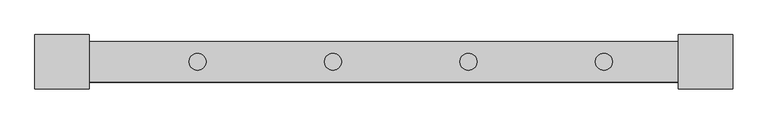
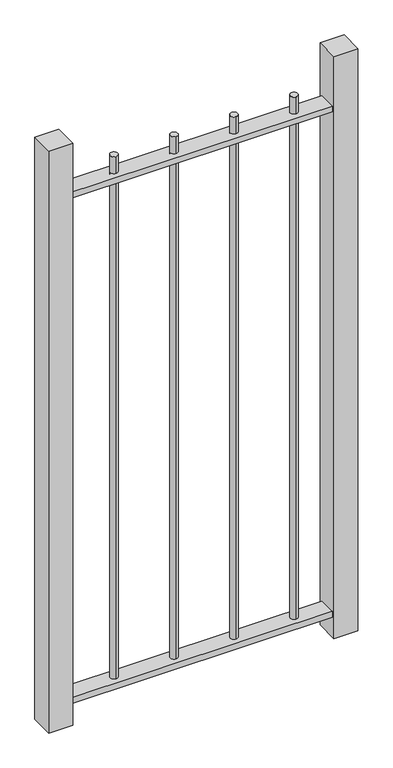
"""IFC4 building model written with IfcOpenShell, lengths in millimetres: railing geometry."""

from ifc_helpers import new_model, si_unit, point, frame, frame_2d, origin, place, context, project, spatial, polyline, circle_curve, trimmed, segment, composite_curve, outline, extrude, source, transform, mapped, element, save


def railing_1dd9141f(model_context):
    return source(origin(), model_context, "Body", "SweptSolid", [
        extrude(outline(polyline([(-6519.419961, -24961.1119119), (-6519.419961, -24901.1119119), (-5569.419961, -24901.1119119), (-5569.419961, -24961.1119119), (-6519.419961, -24961.1119119)])), frame((0.0, 0.0, -30.0), z_axis=(0.0, 0.0, 1.0), x_axis=(1.0, 0.0, 0.0)), (0.0, 0.0, 1.0), 20.0),
        extrude(outline(polyline([(-6519.419961, -24961.1119119), (-6519.419961, -24901.1119119), (-5569.419961, -24901.1119119), (-5569.419961, -24961.1119119), (-6519.419961, -24961.1119119)])), frame((0.0, 0.0, 1750.0), z_axis=(0.0, 0.0, 1.0), x_axis=(1.0, 0.0, 0.0)), (0.0, 0.0, 1.0), 20.0),
        extrude(outline(composite_curve([segment(trimmed(circle_curve(frame_2d((-5719.419961, -24931.1119119)), 12.5), [point((-5719.419961, -24943.6119119))], [point((-5719.419961, -24918.6119119))], False, "CARTESIAN"), True, "CONTINUOUS"), segment(trimmed(circle_curve(frame_2d((-5719.419961, -24931.1119119)), 12.5), [point((-5719.419961, -24918.6119119))], [point((-5719.419961, -24943.6119119))], False, "CARTESIAN"), True, "CONTINUOUS")], self_intersect=False)), frame((0.0, 0.0, -10.0), z_axis=(0.0, 0.0, 1.0), x_axis=(1.0, 0.0, 0.0)), (0.0, 0.0, 1.0), 1840.0),
        extrude(outline(composite_curve([segment(trimmed(circle_curve(frame_2d((-5919.419961, -24931.1119119)), 12.5), [point((-5919.419961, -24943.6119119))], [point((-5919.419961, -24918.6119119))], False, "CARTESIAN"), True, "CONTINUOUS"), segment(trimmed(circle_curve(frame_2d((-5919.419961, -24931.1119119)), 12.5), [point((-5919.419961, -24918.6119119))], [point((-5919.419961, -24943.6119119))], False, "CARTESIAN"), True, "CONTINUOUS")], self_intersect=False)), frame((0.0, 0.0, -10.0), z_axis=(0.0, 0.0, 1.0), x_axis=(1.0, 0.0, 0.0)), (0.0, 0.0, 1.0), 1840.0),
        extrude(outline(composite_curve([segment(trimmed(circle_curve(frame_2d((-6119.419961, -24931.1119119)), 12.5), [point((-6119.419961, -24943.6119119))], [point((-6119.419961, -24918.6119119))], False, "CARTESIAN"), True, "CONTINUOUS"), segment(trimmed(circle_curve(frame_2d((-6119.419961, -24931.1119119)), 12.5), [point((-6119.419961, -24918.6119119))], [point((-6119.419961, -24943.6119119))], False, "CARTESIAN"), True, "CONTINUOUS")], self_intersect=False)), frame((0.0, 0.0, -10.0), z_axis=(0.0, 0.0, 1.0), x_axis=(1.0, 0.0, 0.0)), (0.0, 0.0, 1.0), 1840.0),
        extrude(outline(composite_curve([segment(trimmed(circle_curve(frame_2d((-6319.419961, -24931.1119119)), 12.5), [point((-6319.419961, -24943.6119119))], [point((-6319.419961, -24918.6119119))], False, "CARTESIAN"), True, "CONTINUOUS"), segment(trimmed(circle_curve(frame_2d((-6319.419961, -24931.1119119)), 12.5), [point((-6319.419961, -24918.6119119))], [point((-6319.419961, -24943.6119119))], False, "CARTESIAN"), True, "CONTINUOUS")], self_intersect=False)), frame((0.0, 0.0, -10.0), z_axis=(0.0, 0.0, 1.0), x_axis=(1.0, 0.0, 0.0)), (0.0, 0.0, 1.0), 1840.0),
        extrude(outline(polyline([(-5609.419961, -24891.1119119), (-5529.419961, -24891.1119119), (-5529.419961, -24971.1119119), (-5609.419961, -24971.1119119), (-5609.419961, -24891.1119119)])), frame((0.0, 0.0, -100.0), z_axis=(0.0, 0.0, 1.0), x_axis=(1.0, 0.0, 0.0)), (0.0, 0.0, 1.0), 2050.0),
        extrude(outline(polyline([(-6559.419961, -24891.1119119), (-6479.419961, -24891.1119119), (-6479.419961, -24971.1119119), (-6559.419961, -24971.1119119), (-6559.419961, -24891.1119119)])), frame((0.0, 0.0, -100.0), z_axis=(0.0, 0.0, 1.0), x_axis=(1.0, 0.0, 0.0)), (0.0, 0.0, 1.0), 2050.0),
    ])


if __name__ == "__main__":
    model = new_model("IFC4")
    model_context = context("Model", 3, world=origin())
    ifc_project = project(units=[si_unit("LENGTHUNIT", "METRE", prefix="MILLI")], contexts=[model_context])
    site = spatial("IfcSite", under=ifc_project)
    building = spatial("IfcBuilding", under=site)
    placement = place(None, origin())
    railing_shape = railing_1dd9141f(model_context)
    element("IfcRailing", 1, at=placement, inside=building, context=model_context, shape_type="MappedRepresentation", body=[
        mapped(railing_shape, transform((0.0, 0.0, 0.0), x_axis=(1.0, 0.0, 0.0), y_axis=(0.0, 1.0, 0.0), z_axis=(0.0, 0.0, 1.0))),
    ])
    save(model, "model.ifc")

# Revit data of these elements
# Element 1 (IfcRailing)
#   Materials on its faces: "NLRS_h2_staal_generiek zwart_gen_rsf", "NLRS_h2_staal_gen_rsf"
# Materials
#   "NLRS_h2_staal_generiek zwart_gen_rsf": class "Metal", colour RGB 189 187 185, transparency 0, Manufacturer = "RevitGG", URL = "www.revitgg.nl", Description = "Staal, generiek materiaal", Cost = 0
#   "NLRS_h2_staal_gen_rsf": class "H - Metaal", colour RGB 189 187 185, transparency 0, Keynote = "h2", Model = "generiek", Manufacturer = "Revit Standards Foundation", URL = "www.revitstandards.org", Description = "staal", Cost = 0
